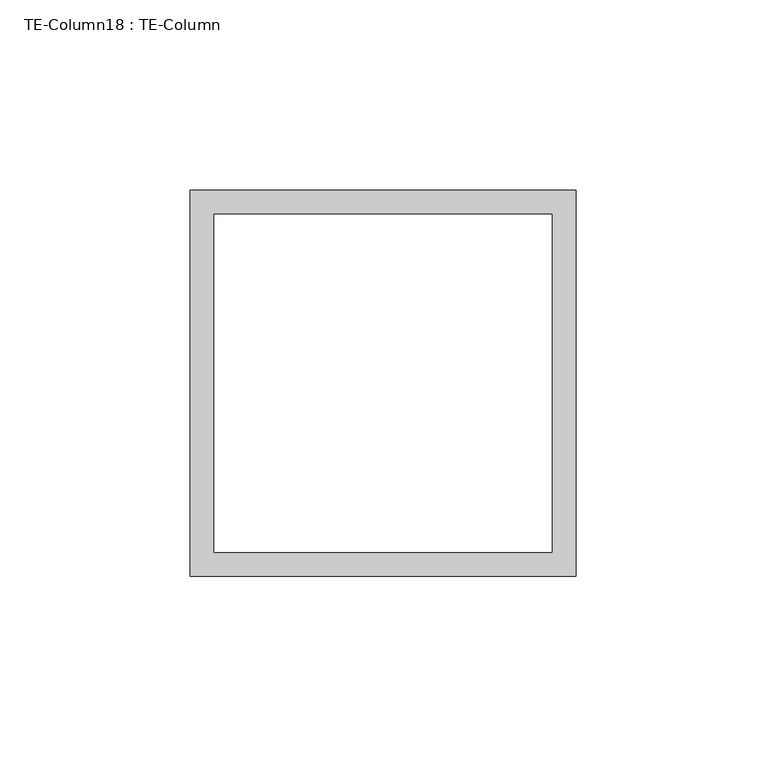
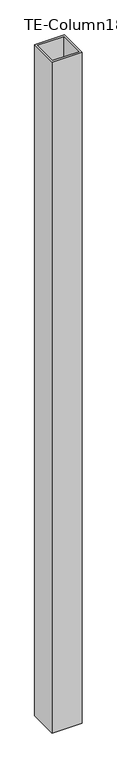
"""IFC4 building model written with IfcOpenShell, lengths in millimetres: proxy geometry, TE-Column18 : TE-Column."""

from ifc_helpers import new_model, si_unit, frame, origin, place, context, project, spatial, polyline, outline, extrude, source, transform, mapped, element, save


def te_column18_te_column_a4862150(model_context):
    return source(origin(), model_context, "Body", "SweptSolid", [
        extrude(outline(polyline([(587365.8934739, -536315.9913841), (587467.4934739, -536315.9913841), (587467.4934739, -536417.5913841), (587365.8934739, -536417.5913841), (587365.8934739, -536315.9913841)]), holes=[polyline([(587372.2434739, -536411.2413841), (587461.1434739, -536411.2413841), (587461.1434739, -536322.3413841), (587372.2434739, -536322.3413841), (587372.2434739, -536411.2413841)])]), frame((0.0, 0.0, 28.575), z_axis=(0.0, 0.0, 1.0), x_axis=(1.0, 0.0, 0.0)), (0.0, 0.0, 1.0), 2406.65),
    ])


if __name__ == "__main__":
    model = new_model("IFC4")
    model_context = context("Model", 3, world=origin())
    ifc_project = project(units=[si_unit("LENGTHUNIT", "METRE", prefix="MILLI")], contexts=[model_context])
    site = spatial("IfcSite", under=ifc_project)
    building = spatial("IfcBuilding", under=site)
    placement = place(None, origin())
    te_column18_te_column_shape = te_column18_te_column_a4862150(model_context)
    element("IfcBuildingElementProxy", 1, Name="TE-Column18 : TE-Column", ObjectType="TE-Column18 : TE-Column", at=placement, inside=building, context=model_context, shape_type="MappedRepresentation", body=[
        mapped(te_column18_te_column_shape, transform((0.0, 0.0, 0.0), x_axis=(1.0, 0.0, 0.0), y_axis=(0.0, 1.0, 0.0), z_axis=(0.0, 0.0, 1.0))),
    ])
    save(model, "model.ifc")

# Revit data of these elements
# Element 1 (IfcBuildingElementProxy, "TE-Column18 : TE-Column")
#   Materials on its faces: "4\"X4\" GALV. HSS TUBING"
# Materials
#   "4\"X4\" GALV. HSS TUBING": class "Generic", colour RGB 211 211 207, transparency 0, Cost = 0
